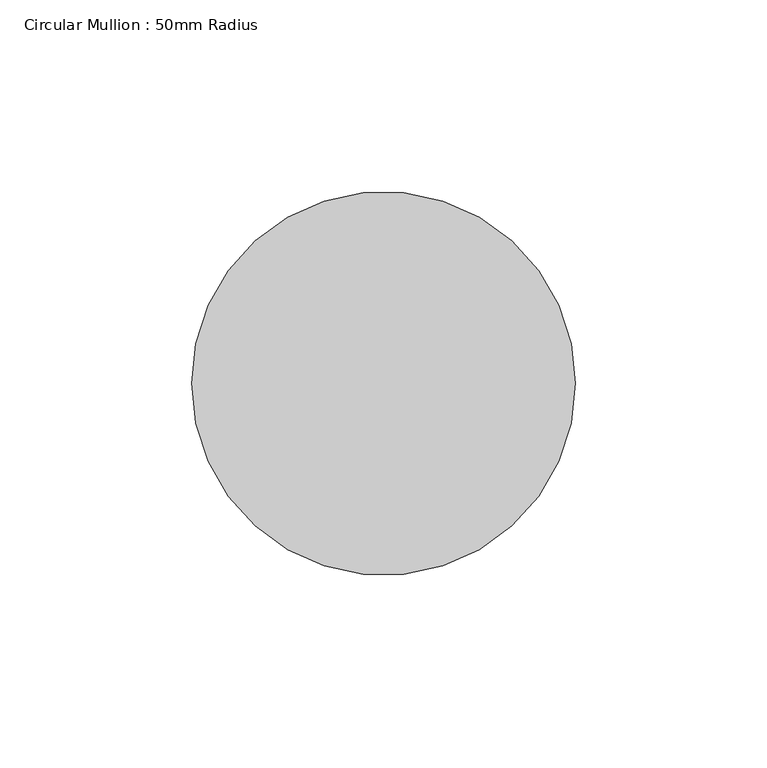
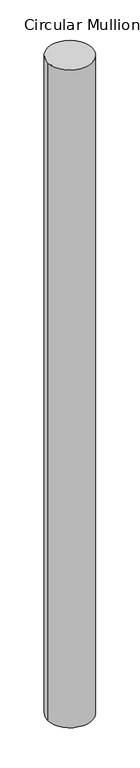
"""IFC4 building model written with IfcOpenShell, lengths in millimetres: member geometry, Circular Mullion : 50mm Radius."""

from ifc_helpers import new_model, si_unit, point, frame, origin, origin_2d, place, context, project, spatial, circle_curve, trimmed, segment, composite_curve, outline, extrude, source, transform, mapped, element, save


def circular_mullion_50mm_radius_5f722388(model_context):
    return source(origin(), model_context, "Body", "SweptSolid", [
        extrude(outline(composite_curve([segment(trimmed(circle_curve(origin_2d(), 50.0), [point((50.0, 0.0))], [point((-50.0, 0.0))], False, "CARTESIAN"), True, "CONTINUOUS"), segment(trimmed(circle_curve(origin_2d(), 50.0), [point((-50.0, 0.0))], [point((50.0, 0.0))], False, "CARTESIAN"), True, "CONTINUOUS")], self_intersect=False)), frame((0.0, 0.0, -1556.2345134), z_axis=(0.0, 0.0, 1.0), x_axis=(1.0, 0.0, 0.0)), (0.0, 0.0, 1.0), 1556.2345134),
    ])


if __name__ == "__main__":
    model = new_model("IFC4")
    model_context = context("Model", 3, world=origin())
    ifc_project = project(units=[si_unit("LENGTHUNIT", "METRE", prefix="MILLI")], contexts=[model_context])
    site = spatial("IfcSite", under=ifc_project)
    building = spatial("IfcBuilding", under=site)
    placement = place(None, origin())
    circular_mullion_50mm_radius_shape = circular_mullion_50mm_radius_5f722388(model_context)
    element("IfcMember", 1, ObjectType="Circular Mullion : 50mm Radius", at=placement, inside=building, context=model_context, shape_type="MappedRepresentation", body=[
        mapped(circular_mullion_50mm_radius_shape, transform((0.0, 0.0, 0.0), x_axis=(1.0, 0.0, 0.0), y_axis=(0.0, 1.0, 0.0), z_axis=(0.0, 0.0, 1.0))),
    ])
    save(model, "model.ifc")

# Revit data of these elements
# Type "Circular Mullion : 50mm Radius"
#   built-in parameter 1007350 = 0.164042 (stored number, unit not read)
# Element 1 (IfcMember, "Circular Mullion : 50mm Radius")
#   Materials on its faces: "Aluminium"
# Materials
#   "Aluminium": class "Metal", colour RGB 247 247 247, transparency 0, Description = "Aluminium 6061", Cost = 0
